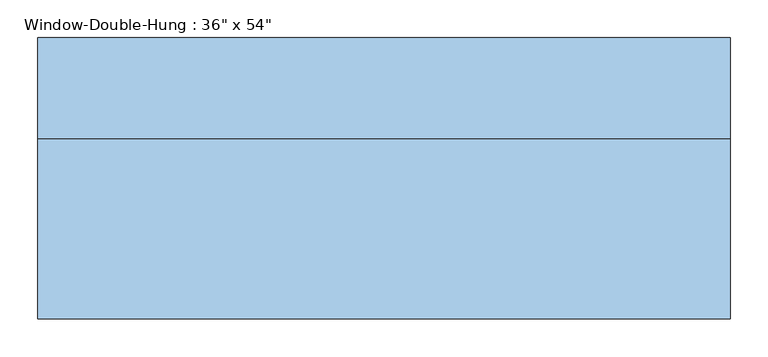
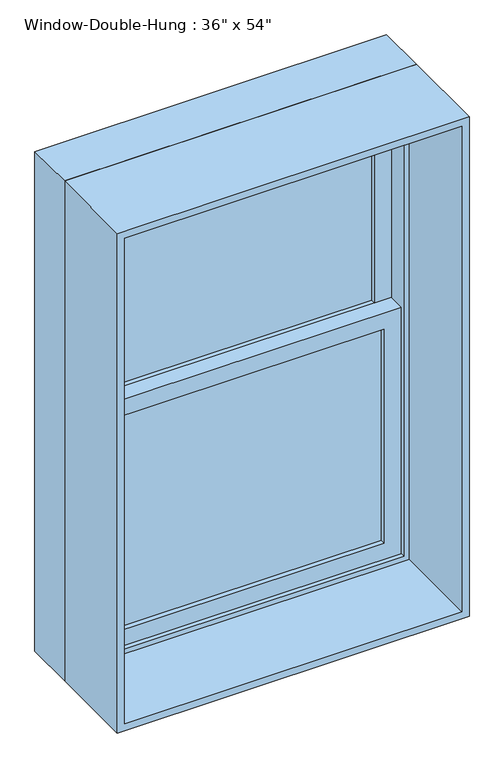
"""IFC4 building model written with IfcOpenShell, lengths in millimetres: window geometry."""

from ifc_helpers import new_model, si_unit, frame, origin, place, context, project, spatial, polyline, outline, extrude, source, transform, mapped, element, save


def window_9f4526fa(model_context):
    return source(origin(), model_context, "Body", "SweptSolid", [
        extrude(outline(polyline([(381.0, 106.3625), (381.0, 100.0125), (-381.0, 100.0125), (-381.0, 106.3625), (381.0, 106.3625)])), frame((0.0, 0.0, 990.6), z_axis=(0.0, 0.0, 1.0), x_axis=(1.0, 0.0, 0.0)), (0.0, 0.0, 1.0), 587.375),
        extrude(outline(polyline([(-381.0, 93.6625), (381.0, 93.6625), (381.0, 87.3125), (-381.0, 87.3125), (-381.0, 93.6625)])), frame((0.0, 0.0, 990.6), z_axis=(0.0, 0.0, 1.0), x_axis=(1.0, 0.0, 0.0)), (0.0, 0.0, 1.0), 587.375),
        extrude(outline(polyline([(381.0, 150.8125), (381.0, 144.4625), (-381.0, 144.4625), (-381.0, 150.8125), (381.0, 150.8125)])), frame((0.0, 0.0, 1622.425), z_axis=(0.0, 0.0, 1.0), x_axis=(1.0, 0.0, 0.0)), (0.0, 0.0, 1.0), 587.375),
        extrude(outline(polyline([(-381.0, 138.1125), (381.0, 138.1125), (381.0, 131.7625), (-381.0, 131.7625), (-381.0, 138.1125)])), frame((0.0, 0.0, 1622.425), z_axis=(0.0, 0.0, 1.0), x_axis=(1.0, 0.0, 0.0)), (0.0, 0.0, 1.0), 587.375),
        extrude(outline(polyline([(1622.425, -425.45), (946.15, -425.45), (946.15, 425.45), (1622.425, 425.45), (1622.425, -425.45)]), holes=[polyline([(1577.975, 381.0), (990.6, 381.0), (990.6, -381.0), (1577.975, -381.0), (1577.975, 381.0)])]), frame((0.0, 74.6125, 0.0), z_axis=(0.0, 1.0, 0.0), x_axis=(0.0, 0.0, 1.0)), (0.0, 0.0, 1.0), 44.45),
        extrude(outline(polyline([(2254.25, -425.45), (1577.975, -425.45), (1577.975, 425.45), (2254.25, 425.45), (2254.25, -425.45)]), holes=[polyline([(2209.8, 381.0), (1622.425, 381.0), (1622.425, -381.0), (2209.8, -381.0), (2209.8, 381.0)])]), frame((0.0, 119.0625, 0.0), z_axis=(0.0, 1.0, 0.0), x_axis=(0.0, 0.0, 1.0)), (0.0, 0.0, 1.0), 44.45),
        extrude(outline(polyline([(2286.0, -457.2), (914.4, -457.2), (914.4, 457.2), (2286.0, 457.2), (2286.0, -457.2)]), holes=[polyline([(2254.25, 425.45), (946.15, 425.45), (946.15, -425.45), (2254.25, -425.45), (2254.25, 425.45)])]), frame((0.0, 61.9125, 0.0), z_axis=(0.0, 1.0, 0.0), x_axis=(0.0, 0.0, 1.0)), (0.0, 0.0, 1.0), 133.35),
        extrude(outline(polyline([(2286.0, 457.2), (2286.0, -457.2), (914.4, -457.2), (914.4, 457.2), (2286.0, 457.2)]), holes=[polyline([(2266.95, 438.15), (933.45, 438.15), (933.45, -438.15), (2266.95, -438.15), (2266.95, 438.15)])]), frame((0.0, -176.2125, 0.0), z_axis=(0.0, 1.0, 0.0), x_axis=(0.0, 0.0, 1.0)), (0.0, 0.0, 1.0), 238.125),
    ])


if __name__ == "__main__":
    model = new_model("IFC4")
    model_context = context("Model", 3, world=origin())
    ifc_project = project(units=[si_unit("LENGTHUNIT", "METRE", prefix="MILLI")], contexts=[model_context])
    site = spatial("IfcSite", under=ifc_project)
    building = spatial("IfcBuilding", under=site)
    placement = place(None, origin())
    window_shape = window_9f4526fa(model_context)
    element("IfcWindow", 1, ObjectType="Window-Double-Hung : 36\" x 54\"", at=placement, inside=building, context=model_context, shape_type="MappedRepresentation", body=[
        mapped(window_shape, transform((0.0, 0.0, 0.0), x_axis=(1.0, 0.0, 0.0), y_axis=(0.0, 1.0, 0.0), z_axis=(0.0, 0.0, 1.0))),
    ])
    save(model, "model.ifc")

# Revit data of these elements
# Type "Window-Double-Hung : 36\" x 54\""
#   Type Mark = "18"
#   Fire Rating = "0.5h"
#   Construction Type Id = "DG-DR"
#   Assembly Code = "B2020100"
#   Analytic Construction = "Double glazing - domestic"
#   Wall Thickness [instance default] = 0' - 6"
#   Window Inset [instance default] = 0' - 0"
#   Visual Light Transmittance = 0.81
#   Thermal Resistance (R) = 1.8146 (h·ft²·°F)/BTU
#   Solar Heat Gain Coefficient = 0.76
#   Muntin Width = 2' - 6"
#   Muntin Height = 1' - 11 1/8"
#   Interior Wall Closure [instance default] = 0' - 1 1/2"
#   Rough Width = 3' - 0 1/2"
#   Rough Height = 4' - 6 1/2"
#   Frame Extension [instance default] = 0' - 1 1/4"
#   Exterior Wall Closure [instance default] = 0' - 0 1/2"
#   Extension Jamb [instance default] = 0' - 1 1/2"
#   Heat Transfer Coefficient (U) = 0.5511 BTU/(h·ft²·°F)
#   Height = 4' - 6"
#   Width = 3' - 0"
#   Top Muntin Visibility = yes
#   Indicator Visibility [instance default] = yes
#   Extension Jamb Visibility [instance default] = yes
#   Interior Trim Visibility [instance default] = yes
#   Exterior Trim Visibility [instance default] = yes
#   Define Thermal Properties by = 1
#   Bottom Muntin Visibility = yes
#   Muntin Pattern = Muntin Pattern_2x2 : Muntin Pattern_2x2
#   Interior Trim Material = Wood - Stained
#   Interior Trim = Trim-Window-Interior-Flat : Picture Frame
#   Exterior Trim Material = Clad - White
#   Exterior Trim = Trim-Window-Exterior-Flat : with Sill
#   Glass Panel Material = Glass
#   Exterior Frame Material = Clad - White
#   Interior Frame Material = Wood - Stained
#   Wall Closure = (empty or 0)
# Element 1 (IfcWindow, "Window-Double-Hung : 36\" x 54\"")
#   Wall Thickness = 1' - 1 7/8"
#   Extension Jamb = 0' - 9 3/8"
#   Materials on its faces: "Wood - Stained", "Glass", "Clad - White"
# Materials
#   "Wood - Stained": class "Wood", colour RGB 224 178 126, transparency 0, Cost = 0
#   "Clad - White": class "Wood", colour RGB 242 242 238, transparency 0, Cost = 0
#   "Glass": class "Glass", colour RGB 0 128 192, transparency 0.75, Description = "Soda Lime Glass", Cost = 0
